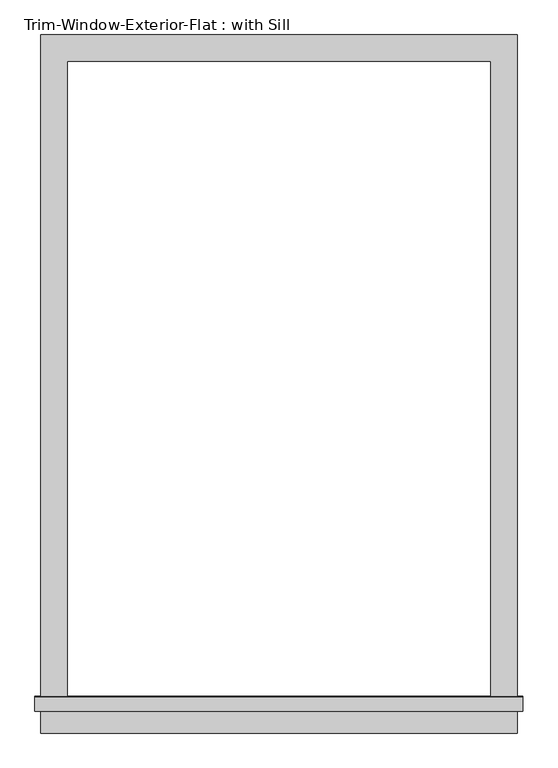
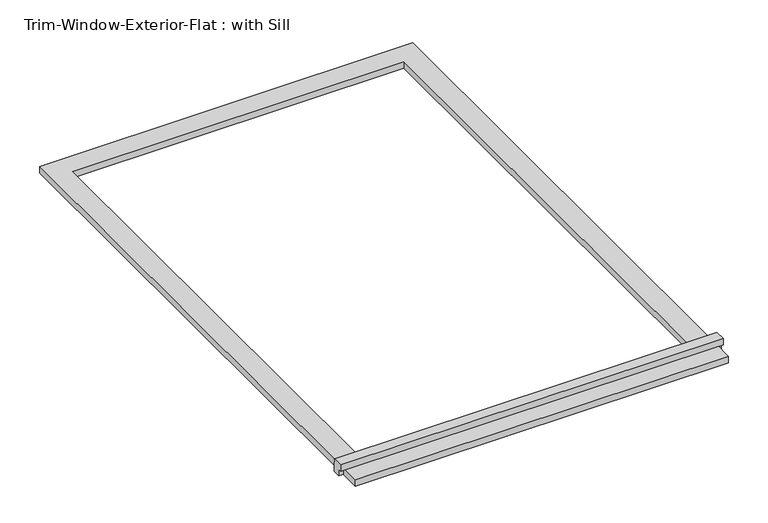
"""IFC4 building model written with IfcOpenShell, lengths in millimetres: proxy geometry, Trim-Window-Exterior-Flat : with Sill."""

from ifc_helpers import new_model, si_unit, frame, origin, origin_with_axes, place, context, project, spatial, polyline, outline, extrude, source, transform, mapped, element, save


def trim_window_exterior_flat_with_sill_8899ae9c(model_context):
    return source(origin(), model_context, "Body", "SweptSolid", [
        extrude(outline(polyline([(514.35, -1393.7823709), (514.35, -1450.9323709), (-514.35, -1450.9323709), (-514.35, -1393.7823709), (514.35, -1393.7823709)])), origin_with_axes(), (0.0, 0.0, 1.0), 19.05),
        extrude(outline(polyline([(-1403.35, 38.1), (-1374.0580645, 38.1), (-1371.6, 19.05), (-1371.6, 0.0), (-1393.7823709, 0.0), (-1393.7823709, 19.05), (-1403.35, 19.05), (-1403.35, 38.1)])), frame((-527.05, 0.0, 0.0), z_axis=(1.0, 0.0, 0.0), x_axis=(0.0, 1.0, 0.0)), (0.0, 0.0, 1.0), 1054.1),
        extrude(outline(polyline([(-514.35, 57.15), (514.35, 57.15), (514.35, -1371.6), (457.2, -1371.6), (457.2, 0.0), (-457.2, 0.0), (-457.2, -1371.6), (-514.35, -1371.6), (-514.35, 57.15)])), origin_with_axes(), (0.0, 0.0, 1.0), 19.05),
    ])


if __name__ == "__main__":
    model = new_model("IFC4")
    model_context = context("Model", 3, world=origin())
    ifc_project = project(units=[si_unit("LENGTHUNIT", "METRE", prefix="MILLI")], contexts=[model_context])
    site = spatial("IfcSite", under=ifc_project)
    building = spatial("IfcBuilding", under=site)
    placement = place(None, origin())
    trim_window_exterior_flat_with_sill_shape = trim_window_exterior_flat_with_sill_8899ae9c(model_context)
    element("IfcBuildingElementProxy", 1, Name="Trim-Window-Exterior-Flat : with Sill", ObjectType="Trim-Window-Exterior-Flat : with Sill", at=placement, inside=building, context=model_context, shape_type="MappedRepresentation", body=[
        mapped(trim_window_exterior_flat_with_sill_shape, transform((0.0, 0.0, 0.0), x_axis=(1.0, 0.0, 0.0), y_axis=(0.0, 1.0, 0.0), z_axis=(0.0, 0.0, 1.0))),
    ])
    save(model, "model.ifc")

# Revit data of these elements
# Type "Trim-Window-Exterior-Flat : with Sill"
#   Trim Width = 0' - 2 1/4"
#   Trim Thickness_Picture Frame = 0' - 1 1/4"
#   Trim Thickness_with Sill = 0' - 0 3/4"
#   Sill Thickness = 0' - 1 1/4"
#   Opening Width [instance default] = 2' - 0"
#   Opening Height [instance default] = 3' - 0"
#   Default Elevation = 4' - 0"
#   Sill = yes
#   Picture Frame = no
#   Trim Material [instance default] = none
# Element 1 (IfcBuildingElementProxy, "Trim-Window-Exterior-Flat : with Sill")
#   Opening Width = 3' - 0"
#   Opening Height = 4' - 6"
#   Trim Material = Clad - White
#   Materials on its faces: "Clad - White"
# Materials
#   "Clad - White": class "Wood", colour RGB 245 245 243, transparency 0, Cost = 0
